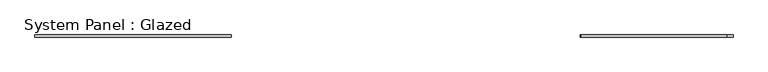
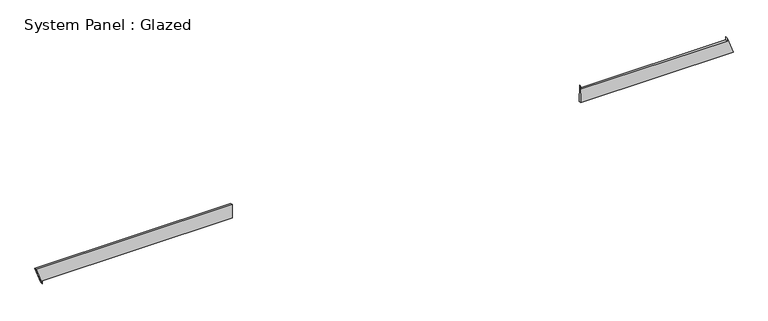
"""IFC4 building model written with IfcOpenShell, lengths in millimetres: plate geometry, System Panel : Glazed."""

from ifc_helpers import new_model, si_unit, frame, origin, place, context, project, spatial, polyline, outline, extrude, source, transform, mapped, element, save


def system_panel_glazed_0fd24995(model_context):
    return source(origin(), model_context, "Body", "SweptSolid", [
        extrude(outline(polyline([(0.0, -3957.0720499), (35.3553391, -3957.0720499), (35.3553391, -1759.4448109), (198.9258324, -1762.342403), (198.9069288, -4026.9181807), (0.0, -3957.0720499)])), frame((0.0, -49.5, 0.0), z_axis=(0.0, 1.0, 0.0), x_axis=(0.0, 0.0, 1.0)), (0.0, 0.0, 1.0), 25.0),
        extrude(outline(polyline([(35.3553391, 2263.6353155), (35.3553391, 4026.9181807), (234.328916, 3957.2301733), (198.9735769, 3957.2304684), (198.9594776, 2268.1982411), (234.3148167, 2268.197946), (35.3553391, 2263.6353155)])), frame((0.0, -49.5, 0.0), z_axis=(0.0, 1.0, 0.0), x_axis=(0.0, 0.0, 1.0)), (0.0, 0.0, 1.0), 25.0),
    ])


if __name__ == "__main__":
    model = new_model("IFC4")
    model_context = context("Model", 3, world=origin())
    ifc_project = project(units=[si_unit("LENGTHUNIT", "METRE", prefix="MILLI")], contexts=[model_context])
    site = spatial("IfcSite", under=ifc_project)
    building = spatial("IfcBuilding", under=site)
    placement = place(None, origin())
    system_panel_glazed_shape = system_panel_glazed_0fd24995(model_context)
    element("IfcPlate", 1, ObjectType="System Panel : Glazed", at=placement, inside=building, context=model_context, shape_type="MappedRepresentation", body=[
        mapped(system_panel_glazed_shape, transform((0.0, 0.0, 0.0), x_axis=(1.0, 0.0, 0.0), y_axis=(0.0, 1.0, 0.0), z_axis=(0.0, 0.0, 1.0))),
    ])
    save(model, "model.ifc")

# Revit data of these elements
# Element 1 (IfcPlate, "System Panel : Glazed")
#   Materials on its faces: "Glass"
# Materials
#   "Glass": class "Glass", colour RGB 218 227 224, transparency 0.85, Description = "Soda Lime Glass", Cost = 0
